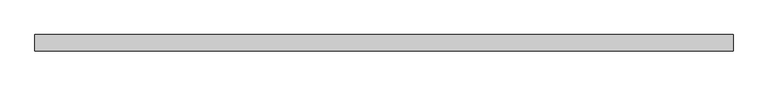
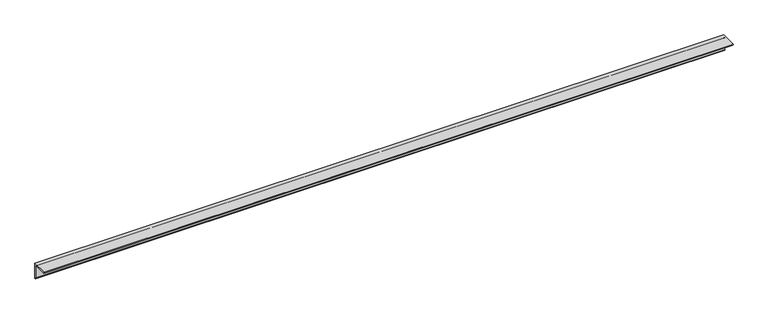
"""IFC4 building model written with IfcOpenShell, lengths in millimetres: member geometry, 0912_Steel Framing_L-KSD3502 : H_SB_AR_S03_L-130x130x12_HBR3."""

from ifc_helpers import new_model, si_unit, point, frame, frame_2d, origin, place, context, project, spatial, polyline, circle_curve, trimmed, segment, composite_curve, outline, extrude, source, transform, mapped, element, save


def member_0cd79b5c(model_context):
    return source(origin(), model_context, "Body", "SweptSolid", [
        extrude(outline(composite_curve([segment(polyline([(36.4, 36.4), (36.4, -93.6)]), True, "CONTINUOUS"), segment(trimmed(circle_curve(frame_2d((36.4, -81.6)), 12.0), [point((36.4, -93.6))], [point((24.4, -81.6))], False, "CARTESIAN"), True, "CONTINUOUS"), segment(polyline([(24.4, -81.6), (24.4, 12.4)]), True, "CONTINUOUS"), segment(trimmed(circle_curve(frame_2d((12.4, 12.4)), 12.0), [point((24.4, 12.4))], [point((12.4, 24.4))], True, "CARTESIAN"), True, "CONTINUOUS"), segment(polyline([(12.4, 24.4), (-81.6, 24.4)]), True, "CONTINUOUS"), segment(trimmed(circle_curve(frame_2d((-81.6, 36.4)), 12.0), [point((-81.6, 24.4))], [point((-93.6, 36.4))], False, "CARTESIAN"), True, "CONTINUOUS"), segment(polyline([(-93.6, 36.4), (36.4, 36.4)]), True, "CONTINUOUS")], self_intersect=False)), frame((-2744.5155402, 0.0, 0.0), z_axis=(1.0, 0.0, 0.0), x_axis=(0.0, 1.0, 0.0)), (0.0, 0.0, 1.0), 5521.206981),
    ])


if __name__ == "__main__":
    model = new_model("IFC4")
    model_context = context("Model", 3, world=origin())
    ifc_project = project(units=[si_unit("LENGTHUNIT", "METRE", prefix="MILLI")], contexts=[model_context])
    site = spatial("IfcSite", under=ifc_project)
    building = spatial("IfcBuilding", under=site)
    placement = place(None, origin())
    member_shape = member_0cd79b5c(model_context)
    element("IfcMember", 1, ObjectType="0912_Steel Framing_L-KSD3502 : H_SB_AR_S03_L-130x130x12_HBR3", at=placement, inside=building, context=model_context, shape_type="MappedRepresentation", body=[
        mapped(member_shape, transform((0.0, 0.0, 0.0), x_axis=(1.0, 0.0, 0.0), y_axis=(0.0, 1.0, 0.0), z_axis=(0.0, 0.0, 1.0))),
    ])
    save(model, "model.ifc")

# Revit data of these elements
# Type "0912_Steel Framing_L-KSD3502 : H_SB_AR_S03_L-130x130x12_HBR3"
#   k = 25 mm
#   Perimeter = 0.52 m²/m
#   Nominal Weight = 23.40 kgf/m
#   Length [instance default] = 1000 mm
#   b = 130 mm
#   d = 130 mm
#   t = 12 mm
#   x = 36.4 mm
#   y = 36.4 mm
#   A = 2976.00 m²
#   Structural Material [instance default] = Steel, 45-345
# Element 1 (IfcMember, "0912_Steel Framing_L-KSD3502 : H_SB_AR_S03_L-130x130x12_HBR3")
#   Structural Material = Steel ASTM A36
#   Materials on its faces: "Steel ASTM A36"
# Materials
#   "Steel, 45-345": class "Metal", colour RGB 189 187 185, transparency 0, Description = "Steel 345 MPa", Cost = 0
#   "Steel ASTM A36": class "Metal", colour RGB 199 199 199, transparency 0, Description = "Structural steel, ASTM A36 Grade B, mill finish", Cost = 0
